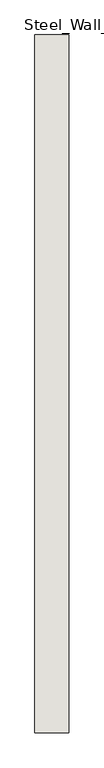
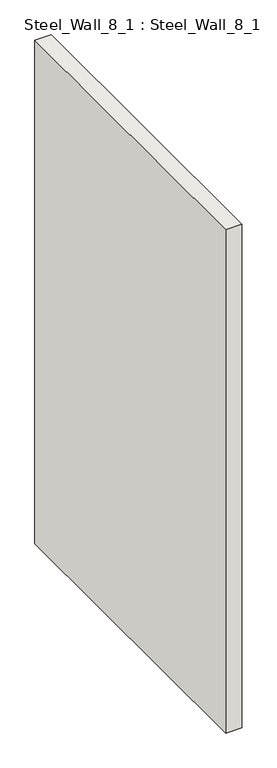
"""IFC4 building model written with IfcOpenShell, lengths in millimetres: wall geometry, Steel_Wall_8_1 : Steel_Wall_8_1."""

from ifc_helpers import new_model, si_unit, frame, origin, place, context, project, spatial, polyline, outline, extrude, source, transform, mapped, element, save


def steel_wall_8_1_steel_wall_8_1_6002a07f(model_context):
    return source(origin(), model_context, "Body", "SweptSolid", [
        extrude(outline(polyline([(6175.0, 16755.0), (6175.0, 14705.0), (6075.0, 14705.0), (6075.0, 16755.0), (6175.0, 16755.0)])), frame((0.0, 0.0, 250.0), z_axis=(0.0, 0.0, 1.0), x_axis=(1.0, 0.0, 0.0)), (0.0, 0.0, 1.0), 3300.0),
    ])


if __name__ == "__main__":
    model = new_model("IFC4")
    model_context = context("Model", 3, world=origin())
    ifc_project = project(units=[si_unit("LENGTHUNIT", "METRE", prefix="MILLI")], contexts=[model_context])
    site = spatial("IfcSite", under=ifc_project)
    building = spatial("IfcBuilding", under=site)
    placement = place(None, origin())
    steel_wall_8_1_steel_wall_8_1_shape = steel_wall_8_1_steel_wall_8_1_6002a07f(model_context)
    element("IfcWall", 1, ObjectType="Steel_Wall_8_1 : Steel_Wall_8_1", at=placement, inside=building, context=model_context, shape_type="MappedRepresentation", body=[
        mapped(steel_wall_8_1_steel_wall_8_1_shape, transform((0.0, 0.0, 0.0), x_axis=(1.0, 0.0, 0.0), y_axis=(0.0, 1.0, 0.0), z_axis=(0.0, 0.0, 1.0))),
    ])
    save(model, "model.ifc")

# Revit data of these elements
# Type "Steel_Wall_8_1 : Steel_Wall_8_1"
#   NameOverride = "Steel_Wall_8_1"
# Element 1 (IfcWall, "Steel_Wall_8_1 : Steel_Wall_8_1")
#   Materials on its faces: "IfcSurfaceStyle #33"
# Materials
#   "IfcSurfaceStyle #33": class "Unassigned", colour RGB 214 214 214, transparency 0
